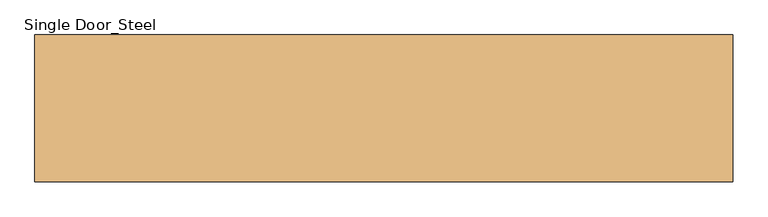
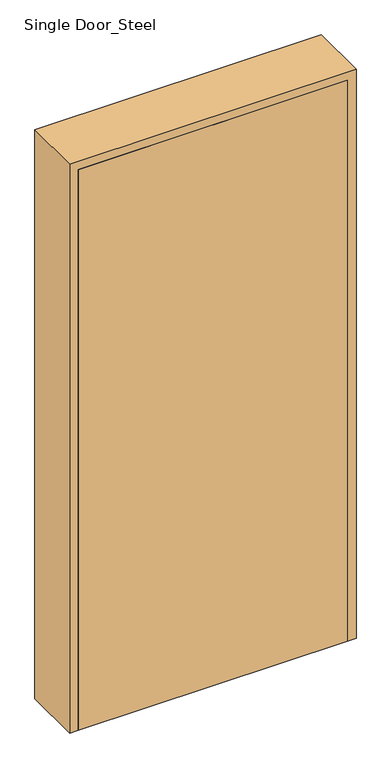
"""IFC4 building model written with IfcOpenShell, lengths in millimetres: door geometry, Single Door_Steel : H_DR_AR_B12_Single Door_Steel_W1000xH2100."""

from ifc_helpers import new_model, si_unit, origin, origin_with_axes, place, context, project, spatial, polyline, outline, extrude, faceted_brep, source, transform, mapped, element, save


def single_door_steel_8d57826b(model_context):
    return source(origin(), model_context, "Body", "SolidModel", [
        extrude(outline(polyline([(470.0, -105.0), (-470.0, -105.0), (-470.0, -70.0), (470.0, -70.0), (470.0, -105.0)])), origin_with_axes(), (0.0, 0.0, 1.0), 2070.0),
        faceted_brep([(470.0, -105.0, 0.0), (470.0, -70.0, 0.0), (450.0, -70.0, 0.0), (450.0, 70.0, 0.0), (470.0, 70.0, 0.0), (470.0, 105.0, 0.0), (500.0, 105.0, 0.0), (500.0, -105.0, 0.0), (500.0, -105.0, 2100.0), (-500.0, -105.0, 2100.0), (-500.0, -105.0, 0.0), (-470.0, -105.0, 0.0), (-470.0, -105.0, 2070.0), (470.0, -105.0, 2070.0), (500.0, 105.0, 2100.0), (470.0, 105.0, 2070.0), (-470.0, 105.0, 2070.0), (-470.0, 105.0, 0.0), (-500.0, 105.0, 0.0), (-500.0, 105.0, 2100.0), (470.0, 70.0, 2070.0), (450.0, 70.0, 2050.0), (-450.0, 70.0, 2050.0), (-450.0, 70.0, 0.0), (-470.0, 70.0, 0.0), (-470.0, 70.0, 2070.0), (450.0, -70.0, 2050.0), (470.0, -70.0, 2070.0), (-470.0, -70.0, 2070.0), (-470.0, -70.0, 0.0), (-450.0, -70.0, 0.0), (-450.0, -70.0, 2050.0)], [[[0, 1, 2, 3, 4, 5, 6, 7]], [[7, 8, 9, 10, 11, 12, 13, 0]], [[6, 14, 8, 7]], [[5, 15, 16, 17, 18, 19, 14, 6]], [[4, 20, 15, 5]], [[3, 21, 22, 23, 24, 25, 20, 4]], [[2, 26, 21, 3]], [[1, 27, 28, 29, 30, 31, 26, 2]], [[0, 13, 27, 1]], [[12, 11, 29, 28]], [[11, 10, 18, 17, 24, 23, 30, 29]], [[19, 18, 10, 9]], [[25, 24, 17, 16]], [[31, 30, 23, 22]], [[14, 19, 9, 8]], [[20, 25, 16, 15]], [[26, 31, 22, 21]], [[13, 12, 28, 27]]]),
    ])


if __name__ == "__main__":
    model = new_model("IFC4")
    model_context = context("Model", 3, world=origin())
    ifc_project = project(units=[si_unit("LENGTHUNIT", "METRE", prefix="MILLI")], contexts=[model_context])
    site = spatial("IfcSite", under=ifc_project)
    building = spatial("IfcBuilding", under=site)
    placement = place(None, origin())
    single_door_steel_shape = single_door_steel_8d57826b(model_context)
    element("IfcDoor", 1, ObjectType="Single Door_Steel : H_DR_AR_B12_Single Door_Steel_W1000xH2100", at=placement, inside=building, context=model_context, shape_type="MappedRepresentation", body=[
        mapped(single_door_steel_shape, transform((0.0, 0.0, 0.0), x_axis=(1.0, 0.0, 0.0), y_axis=(0.0, 1.0, 0.0), z_axis=(0.0, 0.0, 1.0))),
    ])
    save(model, "model.ifc")

# Revit data of these elements
# Type "Single Door_Steel : H_DR_AR_B12_Single Door_Steel_W1000xH2100"
#   Type Mark = "SD"
#   Analytic Construction = "<None>"
#   프레임 투영 외부. = 25 mm
#   프레임 투영 내부. = 25 mm
#   프레임 폭 = 75 mm
#   Height = 2100 mm
#   Width = 1000 mm
#   Define Thermal Properties by = 1
#   문 패널 = none
#   문 프레임 = none
#   Function = (empty or 0)
#   Wall Closure = (empty or 0)
